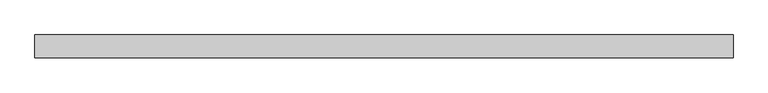
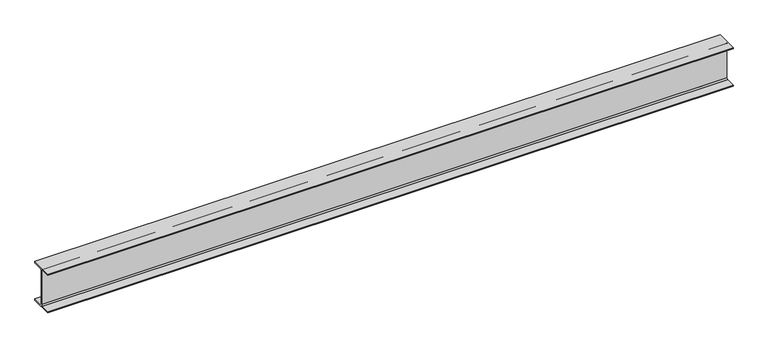
"""IFC4 building model written with IfcOpenShell, lengths in millimetres: beam geometry, Steel Beam_H-KSD3502 : H_SB_ASB_H-300x300x10x15."""

from ifc_helpers import new_model, si_unit, point, frame, frame_2d, origin, place, context, project, spatial, polyline, circle_curve, trimmed, segment, composite_curve, outline, extrude, source, transform, mapped, element, save


def beam_536b1723(model_context):
    return source(origin(), model_context, "Body", "SweptSolid", [
        extrude(outline(composite_curve([segment(polyline([(82.5, -141.5), (82.5, -151.7), (-82.5, -151.7), (-82.5, -141.5), (-11.9, -141.5)]), True, "CONTINUOUS"), segment(trimmed(circle_curve(frame_2d((-11.9, -132.6)), 8.9), [point((-11.9, -141.5))], [point((-3.0, -132.6))], True, "CARTESIAN"), True, "CONTINUOUS"), segment(polyline([(-3.0, -132.6), (-3.0, 132.6)]), True, "CONTINUOUS"), segment(trimmed(circle_curve(frame_2d((-11.9, 132.6)), 8.9), [point((-3.0, 132.6))], [point((-11.9, 141.5))], True, "CARTESIAN"), True, "CONTINUOUS"), segment(polyline([(-11.9, 141.5), (-82.5, 141.5), (-82.5, 151.7), (82.5, 151.7), (82.5, 141.5), (11.9, 141.5)]), True, "CONTINUOUS"), segment(trimmed(circle_curve(frame_2d((11.9, 132.6)), 8.9), [point((11.9, 141.5))], [point((3.0, 132.6))], True, "CARTESIAN"), True, "CONTINUOUS"), segment(polyline([(3.0, 132.6), (3.0, -132.6)]), True, "CONTINUOUS"), segment(trimmed(circle_curve(frame_2d((11.9, -132.6)), 8.9), [point((3.0, -132.6))], [point((11.9, -141.5))], True, "CARTESIAN"), True, "CONTINUOUS"), segment(polyline([(11.9, -141.5), (82.5, -141.5)]), True, "CONTINUOUS")], self_intersect=False)), frame((-2413.6981883, 0.0, 0.0), z_axis=(1.0, 0.0, 0.0), x_axis=(0.0, 1.0, 0.0)), (0.0, 0.0, 1.0), 5076.9152279),
    ])


if __name__ == "__main__":
    model = new_model("IFC4")
    model_context = context("Model", 3, world=origin())
    ifc_project = project(units=[si_unit("LENGTHUNIT", "METRE", prefix="MILLI")], contexts=[model_context])
    site = spatial("IfcSite", under=ifc_project)
    building = spatial("IfcBuilding", under=site)
    placement = place(None, origin())
    beam_shape = beam_536b1723(model_context)
    element("IfcBeam", 1, ObjectType="Steel Beam_H-KSD3502 : H_SB_ASB_H-300x300x10x15", at=placement, inside=building, context=model_context, shape_type="MappedRepresentation", body=[
        mapped(beam_shape, transform((0.0, 0.0, 0.0), x_axis=(1.0, 0.0, 0.0), y_axis=(0.0, 1.0, 0.0), z_axis=(0.0, 0.0, 1.0))),
    ])
    save(model, "model.ifc")

# Revit data of these elements
# Type "Steel Beam_H-KSD3502 : H_SB_ASB_H-300x300x10x15"
#   Width = 30.0 cm
#   Web Thickness = 1.0 cm
#   Web Fillet = 1.8 cm
#   Warping Constant = 1370670.0 cm⁶
#   Torsional Moment of Inertia = 77.00 cm⁴
#   Torsional Modulus = 1.0 cm³
#   Section Area = 119.8 cm²
#   Plastic Modulus weak axis = 684.0 cm³
#   Plastic Modulus strong axis = 1500.0 cm³
#   Perimeter = 1.75 m²/m
#   Nominal Weight = 94.00 kgf/m
#   Moment of Inertia weak axis = 6750.00 cm⁴
#   Moment of Inertia strong axis = 20400.00 cm⁴
#   Height = 30.0 cm
#   Flange Thickness = 1.5 cm
#   Elastic Modulus weak axis = 450.0 cm³
#   Elastic Modulus strong axis = 1360.0 cm³
#   Centroid Vertical = 15.0 cm
#   Centroid Horizontal = 15.0 cm
#   Length [instance default] = 1.5240 m
#   Structural Material [instance default] = Steel, 45-345
#   Assembly Code = ""
# Element 1 (IfcBeam, "Steel Beam_H-KSD3502 : H_SB_ASB_H-300x300x10x15")
#   Structural Material = none
# Materials
#   "Steel, 45-345": class "Metal", colour RGB 189 187 185, transparency 0, Description = "Steel 345 MPa", Cost = 0
